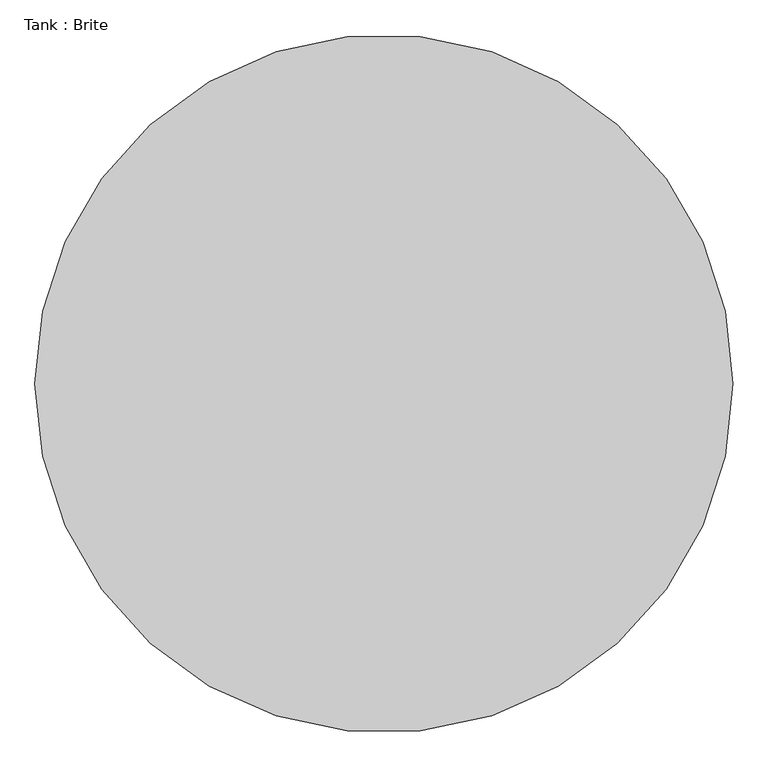
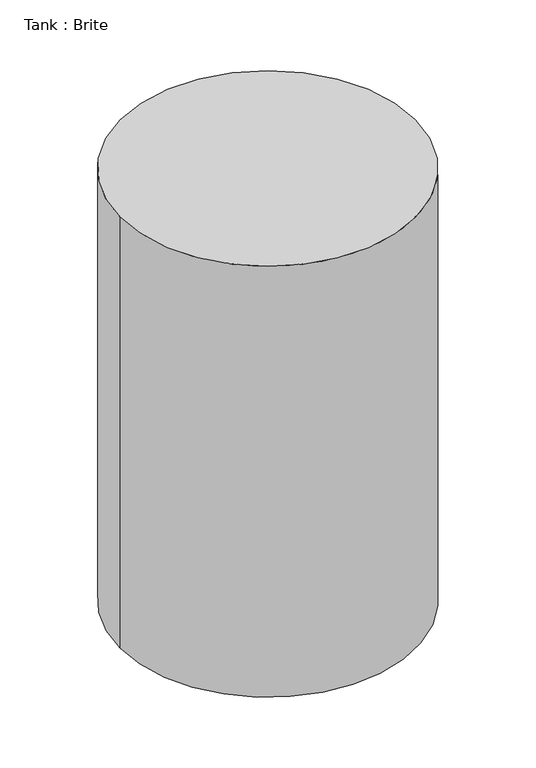
"""IFC4 building model written with IfcOpenShell, lengths in millimetres: proxy geometry, Tank : Brite."""

from ifc_helpers import new_model, si_unit, point, origin, origin_with_axes, origin_2d, place, context, project, spatial, circle_curve, trimmed, segment, composite_curve, outline, extrude, source, transform, mapped, element, save


def tank_brite_224dde2c(model_context):
    return source(origin(), model_context, "Body", "SweptSolid", [
        extrude(outline(composite_curve([segment(trimmed(circle_curve(origin_2d(), 889.0), [point((-889.0, 0.0))], [point((889.0, 0.0))], False, "CARTESIAN"), True, "CONTINUOUS"), segment(trimmed(circle_curve(origin_2d(), 889.0), [point((889.0, 0.0))], [point((-889.0, 0.0))], False, "CARTESIAN"), True, "CONTINUOUS")], self_intersect=False)), origin_with_axes(), (0.0, 0.0, 1.0), 2743.2),
    ])


if __name__ == "__main__":
    model = new_model("IFC4")
    model_context = context("Model", 3, world=origin())
    ifc_project = project(units=[si_unit("LENGTHUNIT", "METRE", prefix="MILLI")], contexts=[model_context])
    site = spatial("IfcSite", under=ifc_project)
    building = spatial("IfcBuilding", under=site)
    placement = place(None, origin())
    tank_brite_shape = tank_brite_224dde2c(model_context)
    element("IfcBuildingElementProxy", 1, Name="Tank : Brite", ObjectType="Tank : Brite", at=placement, inside=building, context=model_context, shape_type="MappedRepresentation", body=[
        mapped(tank_brite_shape, transform((0.0, 0.0, 0.0), x_axis=(1.0, 0.0, 0.0), y_axis=(0.0, 1.0, 0.0), z_axis=(0.0, 0.0, 1.0))),
    ])
    save(model, "model.ifc")

# Revit data of these elements
# Type "Tank : Brite"
#   radius = 2' - 11"
#   Height = 9' - 0"
#   Diameter = 5' - 10"
#   Material = BBT (30 BBL)
# Element 1 (IfcBuildingElementProxy, "Tank : Brite")
#   Materials on its faces: "BBT (30 BBL)"
# Materials
#   "BBT (30 BBL)": class "Generic", colour RGB 181 181 181, transparency 0, Cost = 0
